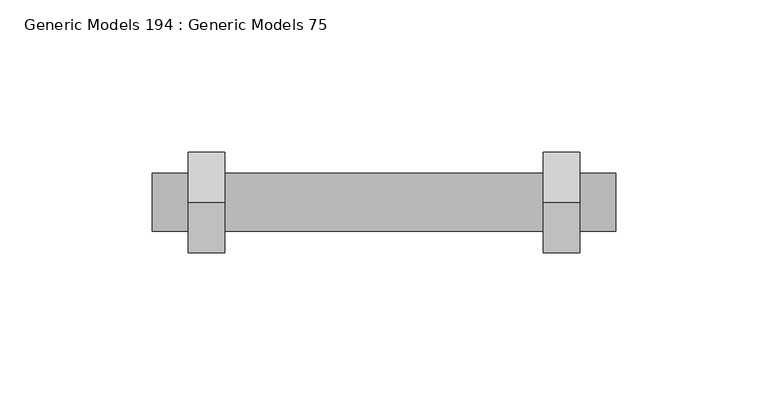
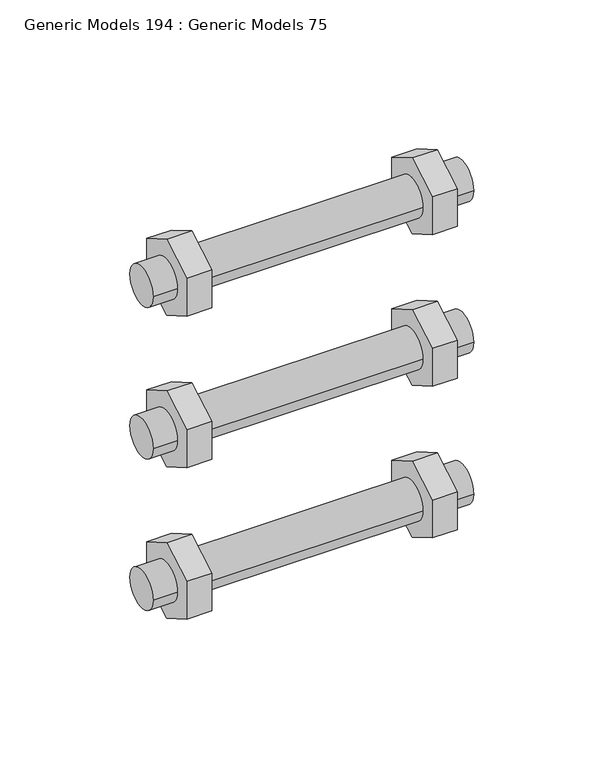
"""IFC4 building model written with IfcOpenShell, lengths in millimetres: proxy geometry, Generic Models 194 : Generic Models 75."""

from ifc_helpers import new_model, si_unit, point, frame, frame_2d, origin, place, context, project, spatial, polyline, circle_curve, trimmed, segment, composite_curve, outline, extrude, source, transform, mapped, element, save


def generic_models_194_generic_models_75_5256b18e(model_context):
    return source(origin(), model_context, "Body", "SweptSolid", [
        extrude(outline(polyline([(35151.5373281, 269062.859622), (35151.5373281, 269043.809622), (35135.0395442, 269034.284622), (35118.5417603, 269043.809622), (35118.5417603, 269062.859622), (35135.0395442, 269072.384622), (35151.5373281, 269062.859622)])), frame((31918.2596032, 0.0, 0.0), z_axis=(1.0, 0.0, 0.0), x_axis=(0.0, 1.0, 0.0)), (0.0, 0.0, 1.0), 11.90625),
        extrude(outline(polyline([(35151.5373281, 268986.659622), (35151.5373281, 268967.609622), (35135.0395442, 268958.084622), (35118.5417603, 268967.609622), (35118.5417603, 268986.659622), (35135.0395442, 268996.184622), (35151.5373281, 268986.659622)])), frame((31918.2596032, 0.0, 0.0), z_axis=(1.0, 0.0, 0.0), x_axis=(0.0, 1.0, 0.0)), (0.0, 0.0, 1.0), 11.90625),
        extrude(outline(polyline([(35151.5373281, 268910.459622), (35151.5373281, 268891.409622), (35135.0395442, 268881.884622), (35118.5417603, 268891.409622), (35118.5417603, 268910.459622), (35135.0395442, 268919.984622), (35151.5373281, 268910.459622)])), frame((31918.2596032, 0.0, 0.0), z_axis=(1.0, 0.0, 0.0), x_axis=(0.0, 1.0, 0.0)), (0.0, 0.0, 1.0), 11.90625),
        extrude(outline(polyline([(35151.5373281, 269062.859622), (35151.5373281, 269043.809622), (35135.0395442, 269034.284622), (35118.5417603, 269043.809622), (35118.5417603, 269062.859622), (35135.0395442, 269072.384622), (35151.5373281, 269062.859622)])), frame((31801.5783532, 0.0, 0.0), z_axis=(1.0, 0.0, 0.0), x_axis=(0.0, 1.0, 0.0)), (0.0, 0.0, 1.0), 11.90625),
        extrude(outline(polyline([(35151.5373281, 268986.659622), (35151.5373281, 268967.609622), (35135.0395442, 268958.084622), (35118.5417603, 268967.609622), (35118.5417603, 268986.659622), (35135.0395442, 268996.184622), (35151.5373281, 268986.659622)])), frame((31801.5783532, 0.0, 0.0), z_axis=(1.0, 0.0, 0.0), x_axis=(0.0, 1.0, 0.0)), (0.0, 0.0, 1.0), 11.90625),
        extrude(outline(polyline([(35151.5373281, 268910.459622), (35151.5373281, 268891.409622), (35135.0395442, 268881.884622), (35118.5417603, 268891.409622), (35118.5417603, 268910.459622), (35135.0395442, 268919.984622), (35151.5373281, 268910.459622)])), frame((31801.5783532, 0.0, 0.0), z_axis=(1.0, 0.0, 0.0), x_axis=(0.0, 1.0, 0.0)), (0.0, 0.0, 1.0), 11.90625),
        extrude(outline(composite_curve([segment(trimmed(circle_curve(frame_2d((35135.0395442, 268977.134622)), 9.525), [point((35125.5145442, 268977.134622))], [point((35144.5645442, 268977.134622))], False, "CARTESIAN"), True, "CONTINUOUS"), segment(trimmed(circle_curve(frame_2d((35135.0395442, 268977.134622)), 9.525), [point((35144.5645442, 268977.134622))], [point((35125.5145442, 268977.134622))], False, "CARTESIAN"), True, "CONTINUOUS")], self_intersect=False)), frame((31789.6721032, 0.0, 0.0), z_axis=(1.0, 0.0, 0.0), x_axis=(0.0, 1.0, 0.0)), (0.0, 0.0, 1.0), 152.4),
        extrude(outline(composite_curve([segment(trimmed(circle_curve(frame_2d((35135.0395442, 268900.934622)), 9.525), [point((35125.5145442, 268900.934622))], [point((35144.5645442, 268900.934622))], False, "CARTESIAN"), True, "CONTINUOUS"), segment(trimmed(circle_curve(frame_2d((35135.0395442, 268900.934622)), 9.525), [point((35144.5645442, 268900.934622))], [point((35125.5145442, 268900.934622))], False, "CARTESIAN"), True, "CONTINUOUS")], self_intersect=False)), frame((31789.6721032, 0.0, 0.0), z_axis=(1.0, 0.0, 0.0), x_axis=(0.0, 1.0, 0.0)), (0.0, 0.0, 1.0), 152.4),
        extrude(outline(composite_curve([segment(trimmed(circle_curve(frame_2d((35135.0395442, 269053.334622)), 9.525), [point((35125.5145442, 269053.334622))], [point((35144.5645442, 269053.334622))], False, "CARTESIAN"), True, "CONTINUOUS"), segment(trimmed(circle_curve(frame_2d((35135.0395442, 269053.334622)), 9.525), [point((35144.5645442, 269053.334622))], [point((35125.5145442, 269053.334622))], False, "CARTESIAN"), True, "CONTINUOUS")], self_intersect=False)), frame((31789.6721032, 0.0, 0.0), z_axis=(1.0, 0.0, 0.0), x_axis=(0.0, 1.0, 0.0)), (0.0, 0.0, 1.0), 152.4),
    ])


if __name__ == "__main__":
    model = new_model("IFC4")
    model_context = context("Model", 3, world=origin())
    ifc_project = project(units=[si_unit("LENGTHUNIT", "METRE", prefix="MILLI")], contexts=[model_context])
    site = spatial("IfcSite", under=ifc_project)
    building = spatial("IfcBuilding", under=site)
    placement = place(None, origin())
    generic_models_194_generic_models_75_shape = generic_models_194_generic_models_75_5256b18e(model_context)
    element("IfcBuildingElementProxy", 1, Name="Generic Models 194 : Generic Models 75", ObjectType="Generic Models 194 : Generic Models 75", at=placement, inside=building, context=model_context, shape_type="MappedRepresentation", body=[
        mapped(generic_models_194_generic_models_75_shape, transform((0.0, 0.0, 0.0), x_axis=(1.0, 0.0, 0.0), y_axis=(0.0, 1.0, 0.0), z_axis=(0.0, 0.0, 1.0))),
    ])
    save(model, "model.ifc")
